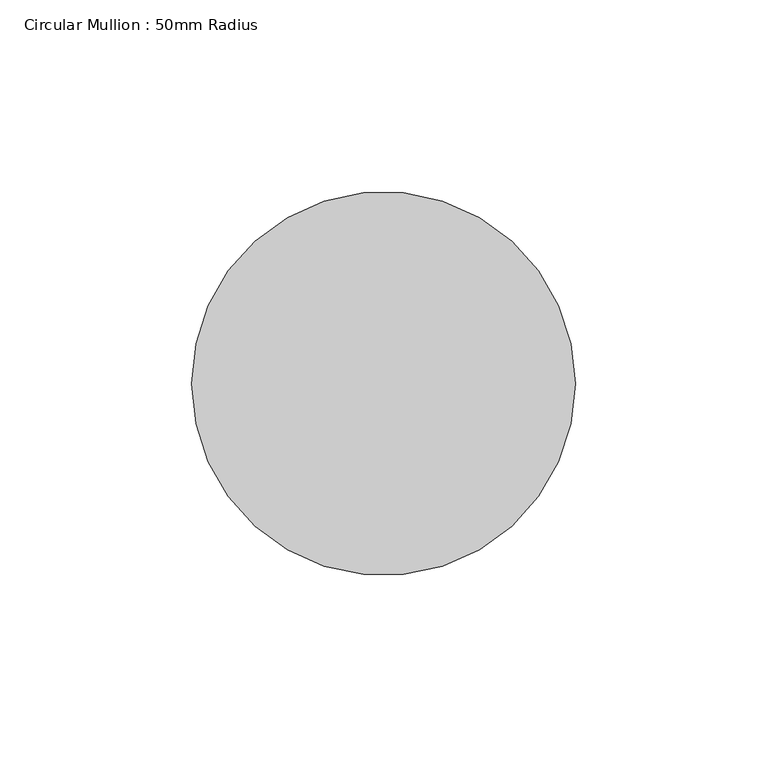
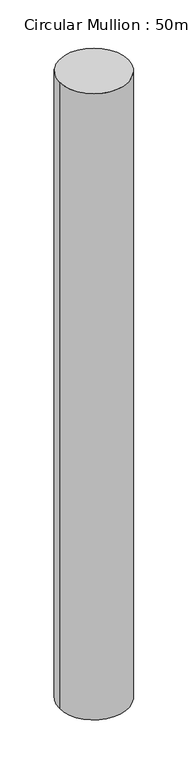
"""IFC4 building model written with IfcOpenShell, lengths in millimetres: member geometry, Circular Mullion : 50mm Radius."""

import ifcopenshell
import ifcopenshell.guid

model = None  # the IFC model being written
_history = None  # IfcOwnerHistory: only IFC2X3 demands one
_inside = {}  # id of a spatial element -> (the spatial element, [elements in it])
_under = {}  # id of a project, library or spatial element -> (it, [spatial elements below it])
_declared = {}  # id of a project -> (the project, [libraries it declares])
_typed = {}  # id of a type object -> (the type object, [elements of that type])
_made_of = {}  # id of a material, layer set ... -> (it, [elements and type objects made of it])


def new_model(schema):
    """Start an empty IFC model of exactly this schema.

    Asked for "IFC4X3", IfcOpenShell would pick the latest addendum, in which some entities
    have other attributes; the version numbers below select the first issue.
    IFC2X3 requires an IfcOwnerHistory on every rooted entity: one is made here for all.
    """
    global model, _history
    if schema == "IFC4X3":
        model = ifcopenshell.file(schema_version=(4, 3, 0, 0))
    else:
        model = ifcopenshell.file(schema=schema)
    _inside.clear()
    _under.clear()
    _declared.clear()
    _typed.clear()
    _made_of.clear()
    _history = None
    if model.schema == "IFC2X3":
        org = make("IfcOrganization", Name="unknown")
        user = make(
            "IfcPersonAndOrganization",
            ThePerson=make("IfcPerson", FamilyName="unknown"),
            TheOrganization=org,
        )
        app = make(
            "IfcApplication",
            ApplicationDeveloper=org,
            Version="unknown",
            ApplicationFullName="unknown",
            ApplicationIdentifier="unknown",
        )
        _history = make(
            "IfcOwnerHistory",
            OwningUser=user,
            OwningApplication=app,
            ChangeAction="ADDED",
            CreationDate=0,
        )
    return model


def make(cls, **values):
    """One entity of the class cls with the attributes given. An attribute that is None is left unset."""
    return model.create_entity(
        cls, **{name: value for name, value in values.items() if value is not None}
    )


def rooted(cls, **values):
    """An entity with a GlobalId (a new one), such as an element, a storey or a relation."""
    return make(cls, GlobalId=ifcopenshell.guid.new(), OwnerHistory=_history, **values)


def si_unit(unit_type, name, prefix=None):
    """IfcSIUnit, for example si_unit("LENGTHUNIT", "METRE", prefix="MILLI")."""
    return make("IfcSIUnit", UnitType=unit_type, Prefix=prefix, Name=name)


def assignment(units):
    """IfcUnitAssignment: the units of a project."""
    return None if units is None else make("IfcUnitAssignment", Units=units)


def point(xyz):
    """IfcCartesianPoint."""
    return None if xyz is None else make("IfcCartesianPoint", Coordinates=xyz)


def direction(xyz):
    """IfcDirection."""
    return None if xyz is None else make("IfcDirection", DirectionRatios=xyz)


def frame(location, z_axis=None, x_axis=None):
    """IfcAxis2Placement3D, a coordinate frame: its origin and axes. An axis left out is left unset."""
    return make(
        "IfcAxis2Placement3D",
        Location=point(location),
        Axis=direction(z_axis),
        RefDirection=direction(x_axis),
    )


def frame_2d(location, x_axis=None):
    """IfcAxis2Placement2D, a coordinate frame in the plane: its origin and x axis."""
    return make(
        "IfcAxis2Placement2D", Location=point(location), RefDirection=direction(x_axis)
    )


def origin():
    """The frame at (0, 0, 0) with its axes left unset."""
    return frame((0.0, 0.0, 0.0))


def origin_2d():
    """The frame at (0, 0) in the plane with its x axis left unset."""
    return frame_2d((0.0, 0.0))


def place(relative_to, where):
    """IfcLocalPlacement: puts the frame where relative to a parent placement (None: the world)."""
    return make(
        "IfcLocalPlacement", PlacementRelTo=relative_to, RelativePlacement=where
    )


def context(
    kind, dimensions, precision=None, world=None, true_north=None, identifier=None
):
    """IfcGeometricRepresentationContext, for example the 3D "Model" context."""
    return make(
        "IfcGeometricRepresentationContext",
        ContextIdentifier=identifier,
        ContextType=kind,
        CoordinateSpaceDimension=dimensions,
        Precision=precision,
        WorldCoordinateSystem=world,
        TrueNorth=true_north,
    )


def project(units=None, contexts=None):
    """IfcProject with its units and contexts."""
    return rooted(
        "IfcProject",
        Name="project",
        RepresentationContexts=contexts,
        UnitsInContext=assignment(units),
    )


def spatial(cls, under=None, at=None, **own):
    """A site, building, storey or space (cls), placed at a placement, below another one or the project."""
    s = rooted(cls, ObjectPlacement=at, **own)
    if under is not None:
        _under.setdefault(under.id(), (under, []))[1].append(s)
    return s


def circle_curve(where, radius):
    """IfcCircle in the frame where."""
    return make("IfcCircle", Position=where, Radius=radius)


def trimmed(basis, trim1, trim2, sense, master):
    """IfcTrimmedCurve: the piece of a basis curve between two trims."""
    return make(
        "IfcTrimmedCurve",
        BasisCurve=basis,
        Trim1=trim1,
        Trim2=trim2,
        SenseAgreement=sense,
        MasterRepresentation=master,
    )


def segment(curve, same_sense, transition):
    """IfcCompositeCurveSegment."""
    return make(
        "IfcCompositeCurveSegment",
        Transition=transition,
        SameSense=same_sense,
        ParentCurve=curve,
    )


def composite_curve(segments, self_intersect=None):
    """IfcCompositeCurve: segments joined end to end."""
    return make("IfcCompositeCurve", Segments=segments, SelfIntersect=self_intersect)


def outline(outer, holes=None, kind="AREA"):
    """IfcArbitraryClosedProfileDef: a profile drawn as a closed curve; with holes, ...WithVoids."""
    if holes is None:
        return make("IfcArbitraryClosedProfileDef", ProfileType=kind, OuterCurve=outer)
    return make(
        "IfcArbitraryProfileDefWithVoids",
        ProfileType=kind,
        OuterCurve=outer,
        InnerCurves=holes,
    )


def extrude(swept, where, along, depth):
    """IfcExtrudedAreaSolid: the profile swept, set in the frame where, extruded along a direction by depth."""
    return make(
        "IfcExtrudedAreaSolid",
        SweptArea=swept,
        Position=where,
        ExtrudedDirection=direction(along),
        Depth=depth,
    )


def shape(context_of_items, identifier, shape_type, items):
    """IfcShapeRepresentation: the items that make up one representation, for example the "Body"."""
    return make(
        "IfcShapeRepresentation",
        ContextOfItems=context_of_items,
        RepresentationIdentifier=identifier,
        RepresentationType=shape_type,
        Items=items,
    )


def source(mapping_origin, context_of_items, identifier, shape_type, items):
    """IfcRepresentationMap: a shape defined once, which mapped items show again and again."""
    return make(
        "IfcRepresentationMap",
        MappingOrigin=mapping_origin,
        MappedRepresentation=shape(context_of_items, identifier, shape_type, items),
    )


def transform(
    local_origin,
    x_axis=None,
    y_axis=None,
    z_axis=None,
    scale=None,
    scale2=None,
    scale3=None,
    uniform=True,
):
    """IfcCartesianTransformationOperator3D, or its non-uniform kind. x_axis, y_axis, z_axis: its Axis1, 2, 3."""
    if uniform:
        return make(
            "IfcCartesianTransformationOperator3D",
            Axis1=direction(x_axis),
            Axis2=direction(y_axis),
            LocalOrigin=point(local_origin),
            Scale=scale,
            Axis3=direction(z_axis),
        )
    return make(
        "IfcCartesianTransformationOperator3DnonUniform",
        Axis1=direction(x_axis),
        Axis2=direction(y_axis),
        LocalOrigin=point(local_origin),
        Scale=scale,
        Axis3=direction(z_axis),
        Scale2=scale2,
        Scale3=scale3,
    )


def mapped(mapping_source, mapping_target):
    """IfcMappedItem: shows the shape of a source again, moved by a transform."""
    return make(
        "IfcMappedItem", MappingSource=mapping_source, MappingTarget=mapping_target
    )


def made_of(thing, what):
    """Note that an element or type object is made of a material, layer set ...; save() writes the relation."""
    if what is not None:
        _made_of.setdefault(what.id(), (what, []))[1].append(thing)
    return thing


def element(
    cls,
    number,
    at=None,
    inside=None,
    cuts=None,
    type_object=None,
    material=None,
    context=None,
    identifier="Body",
    shape_type=None,
    held_by="IfcProductDefinitionShape",
    body=None,
    shapes=None,
    **own,
):
    """One element of the class cls, such as IfcWall. Its Tag is "e" and its number.

    at: its placement. inside: the storey or other place that contains it. cuts: it is an
    opening in that element (IfcRelVoidsElement). A single representation is given by context,
    identifier, shape_type and body (its items); several are given by shapes. held_by: the class
    of the entity that holds the representations. save() writes the other relations.
    """
    e = rooted(cls, Tag="e%d" % number, ObjectPlacement=at, **own)
    if body is not None:
        shapes = [shape(context, identifier, shape_type, body)]
    if shapes is not None:
        e.Representation = make(held_by, Representations=shapes)
    if inside is not None:
        _inside.setdefault(inside.id(), (inside, []))[1].append(e)
    if cuts is not None:
        rooted(
            "IfcRelVoidsElement", RelatingBuildingElement=cuts, RelatedOpeningElement=e
        )
    if type_object is not None:
        _typed.setdefault(type_object.id(), (type_object, []))[1].append(e)
    return made_of(e, material)


def aggregate(whole, parts):
    """IfcRelAggregates: a whole, such as a stair, and the parts it consists of."""
    return rooted("IfcRelAggregates", RelatingObject=whole, RelatedObjects=parts)


def save(model, path):
    """Write the relations noted so far, then the file.

    IfcRelAggregates (storeys below a building ...), IfcRelContainedInSpatialStructure (elements
    in a storey), IfcRelDefinesByType, IfcRelAssociatesMaterial and IfcRelDeclares: one each for
    every whole, place, type object, material and project.
    """
    for whole, parts in _under.values():
        aggregate(whole, parts)
    for where, things in _inside.values():
        rooted(
            "IfcRelContainedInSpatialStructure",
            RelatedElements=things,
            RelatingStructure=where,
        )
    for kind, things in _typed.values():
        rooted("IfcRelDefinesByType", RelatedObjects=things, RelatingType=kind)
    for what, things in _made_of.values():
        rooted("IfcRelAssociatesMaterial", RelatedObjects=things, RelatingMaterial=what)
    for by, libraries in _declared.values():
        rooted("IfcRelDeclares", RelatingContext=by, RelatedDefinitions=libraries)
    model.write(path)


def circular_mullion_50mm_radius_b657400b(model_context):
    return source(origin(), model_context, "Body", "SweptSolid", [
        extrude(outline(composite_curve([segment(trimmed(circle_curve(origin_2d(), 50.0), [point((50.0, 0.0))], [point((-50.0, 0.0))], False, "CARTESIAN"), True, "CONTINUOUS"), segment(trimmed(circle_curve(origin_2d(), 50.0), [point((-50.0, 0.0))], [point((50.0, 0.0))], False, "CARTESIAN"), True, "CONTINUOUS")], self_intersect=False)), frame((0.0, 0.0, -961.1465817), z_axis=(0.0, 0.0, 1.0), x_axis=(1.0, 0.0, 0.0)), (0.0, 0.0, 1.0), 961.1465817),
    ])


if __name__ == "__main__":
    model = new_model("IFC4")
    model_context = context("Model", 3, world=origin())
    ifc_project = project(units=[si_unit("LENGTHUNIT", "METRE", prefix="MILLI")], contexts=[model_context])
    site = spatial("IfcSite", under=ifc_project)
    building = spatial("IfcBuilding", under=site)
    placement = place(None, origin())
    circular_mullion_50mm_radius_shape = circular_mullion_50mm_radius_b657400b(model_context)
    element("IfcMember", 1, ObjectType="Circular Mullion : 50mm Radius", at=placement, inside=building, context=model_context, shape_type="MappedRepresentation", body=[
        mapped(circular_mullion_50mm_radius_shape, transform((0.0, 0.0, 0.0), x_axis=(1.0, 0.0, 0.0), y_axis=(0.0, 1.0, 0.0), z_axis=(0.0, 0.0, 1.0))),
    ])
    save(model, "model.ifc")

# Revit data of these elements
# Type "Circular Mullion : 50mm Radius"
#   built-in parameter 1007350 = 0.164042 (stored number, unit not read)
# Element 1 (IfcMember, "Circular Mullion : 50mm Radius")
#   Materials on its faces: "Aluminium"
# Materials
#   "Aluminium": class "Metal", colour RGB 247 247 247, transparency 0, Description = "Aluminium 6061", Cost = 0
